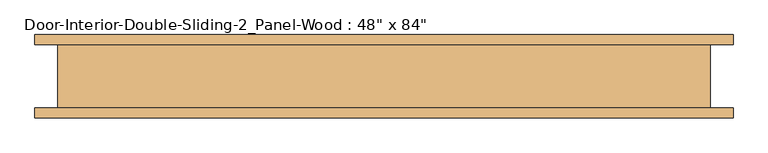
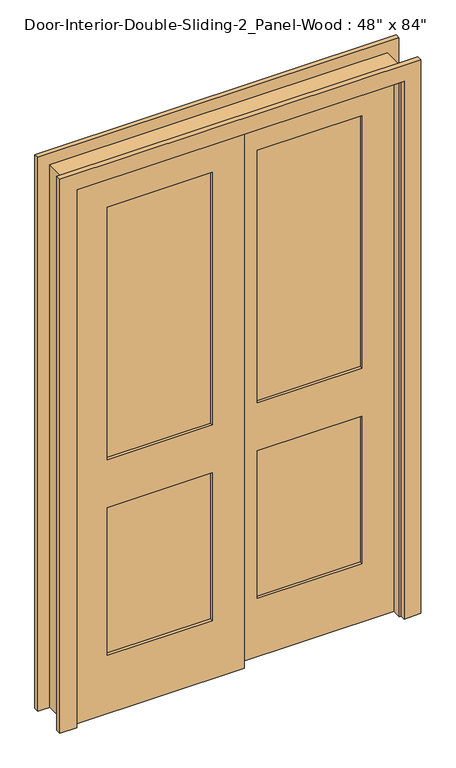
"""IFC4 building model written with IfcOpenShell, lengths in millimetres: door geometry."""

import ifcopenshell
import ifcopenshell.guid

model = None  # the IFC model being written
_history = None  # IfcOwnerHistory: only IFC2X3 demands one
_inside = {}  # id of a spatial element -> (the spatial element, [elements in it])
_under = {}  # id of a project, library or spatial element -> (it, [spatial elements below it])
_declared = {}  # id of a project -> (the project, [libraries it declares])
_typed = {}  # id of a type object -> (the type object, [elements of that type])
_made_of = {}  # id of a material, layer set ... -> (it, [elements and type objects made of it])


def new_model(schema):
    """Start an empty IFC model of exactly this schema.

    Asked for "IFC4X3", IfcOpenShell would pick the latest addendum, in which some entities
    have other attributes; the version numbers below select the first issue.
    IFC2X3 requires an IfcOwnerHistory on every rooted entity: one is made here for all.
    """
    global model, _history
    if schema == "IFC4X3":
        model = ifcopenshell.file(schema_version=(4, 3, 0, 0))
    else:
        model = ifcopenshell.file(schema=schema)
    _inside.clear()
    _under.clear()
    _declared.clear()
    _typed.clear()
    _made_of.clear()
    _history = None
    if model.schema == "IFC2X3":
        org = make("IfcOrganization", Name="unknown")
        user = make(
            "IfcPersonAndOrganization",
            ThePerson=make("IfcPerson", FamilyName="unknown"),
            TheOrganization=org,
        )
        app = make(
            "IfcApplication",
            ApplicationDeveloper=org,
            Version="unknown",
            ApplicationFullName="unknown",
            ApplicationIdentifier="unknown",
        )
        _history = make(
            "IfcOwnerHistory",
            OwningUser=user,
            OwningApplication=app,
            ChangeAction="ADDED",
            CreationDate=0,
        )
    return model


def make(cls, **values):
    """One entity of the class cls with the attributes given. An attribute that is None is left unset."""
    return model.create_entity(
        cls, **{name: value for name, value in values.items() if value is not None}
    )


def rooted(cls, **values):
    """An entity with a GlobalId (a new one), such as an element, a storey or a relation."""
    return make(cls, GlobalId=ifcopenshell.guid.new(), OwnerHistory=_history, **values)


def si_unit(unit_type, name, prefix=None):
    """IfcSIUnit, for example si_unit("LENGTHUNIT", "METRE", prefix="MILLI")."""
    return make("IfcSIUnit", UnitType=unit_type, Prefix=prefix, Name=name)


def assignment(units):
    """IfcUnitAssignment: the units of a project."""
    return None if units is None else make("IfcUnitAssignment", Units=units)


def point(xyz):
    """IfcCartesianPoint."""
    return None if xyz is None else make("IfcCartesianPoint", Coordinates=xyz)


def direction(xyz):
    """IfcDirection."""
    return None if xyz is None else make("IfcDirection", DirectionRatios=xyz)


def frame(location, z_axis=None, x_axis=None):
    """IfcAxis2Placement3D, a coordinate frame: its origin and axes. An axis left out is left unset."""
    return make(
        "IfcAxis2Placement3D",
        Location=point(location),
        Axis=direction(z_axis),
        RefDirection=direction(x_axis),
    )


def origin():
    """The frame at (0, 0, 0) with its axes left unset."""
    return frame((0.0, 0.0, 0.0))


def place(relative_to, where):
    """IfcLocalPlacement: puts the frame where relative to a parent placement (None: the world)."""
    return make(
        "IfcLocalPlacement", PlacementRelTo=relative_to, RelativePlacement=where
    )


def context(
    kind, dimensions, precision=None, world=None, true_north=None, identifier=None
):
    """IfcGeometricRepresentationContext, for example the 3D "Model" context."""
    return make(
        "IfcGeometricRepresentationContext",
        ContextIdentifier=identifier,
        ContextType=kind,
        CoordinateSpaceDimension=dimensions,
        Precision=precision,
        WorldCoordinateSystem=world,
        TrueNorth=true_north,
    )


def project(units=None, contexts=None):
    """IfcProject with its units and contexts."""
    return rooted(
        "IfcProject",
        Name="project",
        RepresentationContexts=contexts,
        UnitsInContext=assignment(units),
    )


def spatial(cls, under=None, at=None, **own):
    """A site, building, storey or space (cls), placed at a placement, below another one or the project."""
    s = rooted(cls, ObjectPlacement=at, **own)
    if under is not None:
        _under.setdefault(under.id(), (under, []))[1].append(s)
    return s


def polyline(points):
    """IfcPolyline through the points."""
    return make("IfcPolyline", Points=[point(p) for p in points])


def outline(outer, holes=None, kind="AREA"):
    """IfcArbitraryClosedProfileDef: a profile drawn as a closed curve; with holes, ...WithVoids."""
    if holes is None:
        return make("IfcArbitraryClosedProfileDef", ProfileType=kind, OuterCurve=outer)
    return make(
        "IfcArbitraryProfileDefWithVoids",
        ProfileType=kind,
        OuterCurve=outer,
        InnerCurves=holes,
    )


def extrude(swept, where, along, depth):
    """IfcExtrudedAreaSolid: the profile swept, set in the frame where, extruded along a direction by depth."""
    return make(
        "IfcExtrudedAreaSolid",
        SweptArea=swept,
        Position=where,
        ExtrudedDirection=direction(along),
        Depth=depth,
    )


def shape(context_of_items, identifier, shape_type, items):
    """IfcShapeRepresentation: the items that make up one representation, for example the "Body"."""
    return make(
        "IfcShapeRepresentation",
        ContextOfItems=context_of_items,
        RepresentationIdentifier=identifier,
        RepresentationType=shape_type,
        Items=items,
    )


def source(mapping_origin, context_of_items, identifier, shape_type, items):
    """IfcRepresentationMap: a shape defined once, which mapped items show again and again."""
    return make(
        "IfcRepresentationMap",
        MappingOrigin=mapping_origin,
        MappedRepresentation=shape(context_of_items, identifier, shape_type, items),
    )


def transform(
    local_origin,
    x_axis=None,
    y_axis=None,
    z_axis=None,
    scale=None,
    scale2=None,
    scale3=None,
    uniform=True,
):
    """IfcCartesianTransformationOperator3D, or its non-uniform kind. x_axis, y_axis, z_axis: its Axis1, 2, 3."""
    if uniform:
        return make(
            "IfcCartesianTransformationOperator3D",
            Axis1=direction(x_axis),
            Axis2=direction(y_axis),
            LocalOrigin=point(local_origin),
            Scale=scale,
            Axis3=direction(z_axis),
        )
    return make(
        "IfcCartesianTransformationOperator3DnonUniform",
        Axis1=direction(x_axis),
        Axis2=direction(y_axis),
        LocalOrigin=point(local_origin),
        Scale=scale,
        Axis3=direction(z_axis),
        Scale2=scale2,
        Scale3=scale3,
    )


def mapped(mapping_source, mapping_target):
    """IfcMappedItem: shows the shape of a source again, moved by a transform."""
    return make(
        "IfcMappedItem", MappingSource=mapping_source, MappingTarget=mapping_target
    )


def made_of(thing, what):
    """Note that an element or type object is made of a material, layer set ...; save() writes the relation."""
    if what is not None:
        _made_of.setdefault(what.id(), (what, []))[1].append(thing)
    return thing


def element(
    cls,
    number,
    at=None,
    inside=None,
    cuts=None,
    type_object=None,
    material=None,
    context=None,
    identifier="Body",
    shape_type=None,
    held_by="IfcProductDefinitionShape",
    body=None,
    shapes=None,
    **own,
):
    """One element of the class cls, such as IfcWall. Its Tag is "e" and its number.

    at: its placement. inside: the storey or other place that contains it. cuts: it is an
    opening in that element (IfcRelVoidsElement). A single representation is given by context,
    identifier, shape_type and body (its items); several are given by shapes. held_by: the class
    of the entity that holds the representations. save() writes the other relations.
    """
    e = rooted(cls, Tag="e%d" % number, ObjectPlacement=at, **own)
    if body is not None:
        shapes = [shape(context, identifier, shape_type, body)]
    if shapes is not None:
        e.Representation = make(held_by, Representations=shapes)
    if inside is not None:
        _inside.setdefault(inside.id(), (inside, []))[1].append(e)
    if cuts is not None:
        rooted(
            "IfcRelVoidsElement", RelatingBuildingElement=cuts, RelatedOpeningElement=e
        )
    if type_object is not None:
        _typed.setdefault(type_object.id(), (type_object, []))[1].append(e)
    return made_of(e, material)


def aggregate(whole, parts):
    """IfcRelAggregates: a whole, such as a stair, and the parts it consists of."""
    return rooted("IfcRelAggregates", RelatingObject=whole, RelatedObjects=parts)


def save(model, path):
    """Write the relations noted so far, then the file.

    IfcRelAggregates (storeys below a building ...), IfcRelContainedInSpatialStructure (elements
    in a storey), IfcRelDefinesByType, IfcRelAssociatesMaterial and IfcRelDeclares: one each for
    every whole, place, type object, material and project.
    """
    for whole, parts in _under.values():
        aggregate(whole, parts)
    for where, things in _inside.values():
        rooted(
            "IfcRelContainedInSpatialStructure",
            RelatedElements=things,
            RelatingStructure=where,
        )
    for kind, things in _typed.values():
        rooted("IfcRelDefinesByType", RelatedObjects=things, RelatingType=kind)
    for what, things in _made_of.values():
        rooted("IfcRelAssociatesMaterial", RelatedObjects=things, RelatingMaterial=what)
    for by, libraries in _declared.values():
        rooted("IfcRelDeclares", RelatingContext=by, RelatedDefinitions=libraries)
    model.write(path)


def door_b8c0c601(model_context):
    return source(origin(), model_context, "Body", "SweptSolid", [
        extrude(outline(polyline([(488.95, -0.5291667), (488.95, -12.1708333), (95.25, -12.1708333), (95.25, -0.5291667), (488.95, -0.5291667)])), frame((0.0, 0.0, 1009.65), z_axis=(0.0, 0.0, 1.0), x_axis=(1.0, 0.0, 0.0)), (0.0, 0.0, 1.0), 1004.8875),
        extrude(outline(polyline([(488.95, -0.5291667), (488.95, -12.1708333), (95.25, -12.1708333), (95.25, -0.5291667), (488.95, -0.5291667)])), frame((0.0, 0.0, 231.775), z_axis=(0.0, 0.0, 1.0), x_axis=(1.0, 0.0, 0.0)), (0.0, 0.0, 1.0), 587.375),
        extrude(outline(polyline([(2133.6, -25.4), (0.0, -25.4), (0.0, 609.6), (2133.6, 609.6), (2133.6, -25.4)]), holes=[polyline([(2014.5375, 95.25), (2014.5375, 488.95), (1009.65, 488.95), (1009.65, 95.25), (2014.5375, 95.25)]), polyline([(819.15, 95.25), (819.15, 488.95), (231.775, 488.95), (231.775, 95.25), (819.15, 95.25)])]), frame((0.0, -23.8125, 0.0), z_axis=(0.0, 1.0, 0.0), x_axis=(0.0, 0.0, 1.0)), (0.0, 0.0, 1.0), 34.925),
        extrude(outline(polyline([(-95.25, -35.4541667), (-95.25, -47.0958333), (-488.95, -47.0958333), (-488.95, -35.4541667), (-95.25, -35.4541667)])), frame((0.0, 0.0, 1009.65), z_axis=(0.0, 0.0, 1.0), x_axis=(1.0, 0.0, 0.0)), (0.0, 0.0, 1.0), 1004.8875),
        extrude(outline(polyline([(-95.25, -35.4541667), (-95.25, -47.0958333), (-488.95, -47.0958333), (-488.95, -35.4541667), (-95.25, -35.4541667)])), frame((0.0, 0.0, 231.775), z_axis=(0.0, 0.0, 1.0), x_axis=(1.0, 0.0, 0.0)), (0.0, 0.0, 1.0), 587.375),
        extrude(outline(polyline([(2133.6, -609.6), (0.0, -609.6), (0.0, 25.4), (2133.6, 25.4), (2133.6, -609.6)]), holes=[polyline([(2014.5375, -488.95), (2014.5375, -95.25), (1009.65, -95.25), (1009.65, -488.95), (2014.5375, -488.95)]), polyline([(819.15, -488.95), (819.15, -95.25), (231.775, -95.25), (231.775, -488.95), (819.15, -488.95)])]), frame((0.0, -58.7375, 0.0), z_axis=(0.0, 1.0, 0.0), x_axis=(0.0, 0.0, 1.0)), (0.0, 0.0, 1.0), 34.925),
        extrude(outline(polyline([(0.0, 635.0), (2159.0, 635.0), (2159.0, -635.0), (0.0, -635.0), (0.0, -609.6), (2133.6, -609.6), (2133.6, 609.6), (0.0, 609.6), (0.0, 635.0)])), frame((0.0, -58.7375, 0.0), z_axis=(0.0, 1.0, 0.0), x_axis=(0.0, 0.0, 1.0)), (0.0, 0.0, 1.0), 123.825),
        extrude(outline(polyline([(0.0, 679.45), (2203.45, 679.45), (2203.45, -679.45), (0.0, -679.45), (0.0, -615.95), (2139.95, -615.95), (2139.95, 615.95), (0.0, 615.95), (0.0, 679.45)])), frame((0.0, 65.0875, 0.0), z_axis=(0.0, 1.0, 0.0), x_axis=(0.0, 0.0, 1.0)), (0.0, 0.0, 1.0), 19.05),
        extrude(outline(polyline([(0.0, 679.45), (2203.45, 679.45), (2203.45, -679.45), (0.0, -679.45), (0.0, -615.95), (2139.95, -615.95), (2139.95, 615.95), (0.0, 615.95), (0.0, 679.45)])), frame((0.0, -77.7875, 0.0), z_axis=(0.0, 1.0, 0.0), x_axis=(0.0, 0.0, 1.0)), (0.0, 0.0, 1.0), 19.05),
    ])


if __name__ == "__main__":
    model = new_model("IFC4")
    model_context = context("Model", 3, world=origin())
    ifc_project = project(units=[si_unit("LENGTHUNIT", "METRE", prefix="MILLI")], contexts=[model_context])
    site = spatial("IfcSite", under=ifc_project)
    building = spatial("IfcBuilding", under=site)
    placement = place(None, origin())
    door_shape = door_b8c0c601(model_context)
    element("IfcDoor", 1, ObjectType="Door-Interior-Double-Sliding-2_Panel-Wood : 48\" x 84\"", at=placement, inside=building, context=model_context, shape_type="MappedRepresentation", body=[
        mapped(door_shape, transform((0.0, 0.0, 0.0), x_axis=(1.0, 0.0, 0.0), y_axis=(0.0, 1.0, 0.0), z_axis=(0.0, 0.0, 1.0))),
    ])
    save(model, "model.ifc")

# Revit data of these elements
# Type "Door-Interior-Double-Sliding-2_Panel-Wood : 48\" x 84\""
#   Type Mark = "21"
#   Assembly Code = "C1020300"
#   Analytic Construction = "Wooden"
#   Top Rail = 0' - 4 11/16"
#   Thickness = 0' - 1 3/8"
#   Thermal Resistance (R) = 2.5876 (h·ft²·°F)/BTU
#   Stiles = 0' - 4 3/4"
#   Rough Width = 4' - 2"
#   Rough Height = 7' - 1"
#   Lock Rail = 0' - 7 1/2"
#   Height = 7' - 0"
#   Width = 4' - 0"
#   Heat Transfer Coefficient (U) = 0.3865 BTU/(h·ft²·°F)
#   Bottom Rail = 0' - 9 1/8"
#   Trim Material = Cherry
#   Panel Material = Cherry
#   Frame Material = Cherry
#   Visual Light Transmittance = 0
#   Solar Heat Gain Coefficient = 0
#   Wall Closure = (empty or 0)
#   Function = (empty or 0)
# Element 1 (IfcDoor, "Door-Interior-Double-Sliding-2_Panel-Wood : 48\" x 84\"")
#   Materials on its faces: "Cherry"
# Materials
#   "Cherry": class "Wood", colour RGB 226 177 128, transparency 0, Description = "Prunus Serotina", Cost = 0
